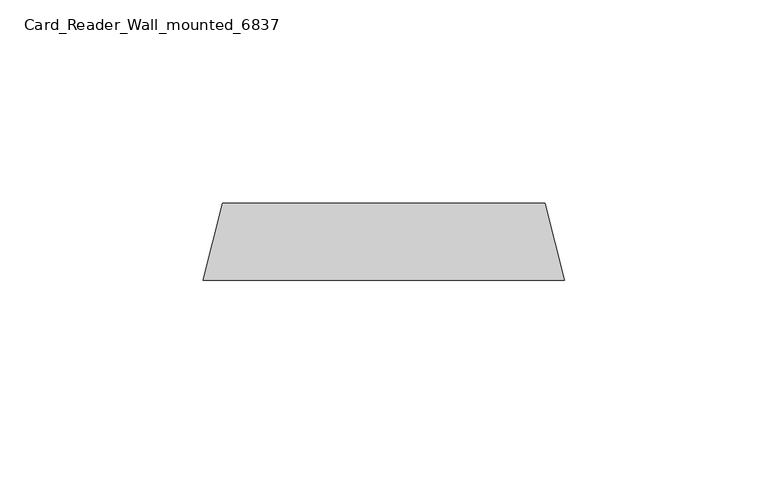
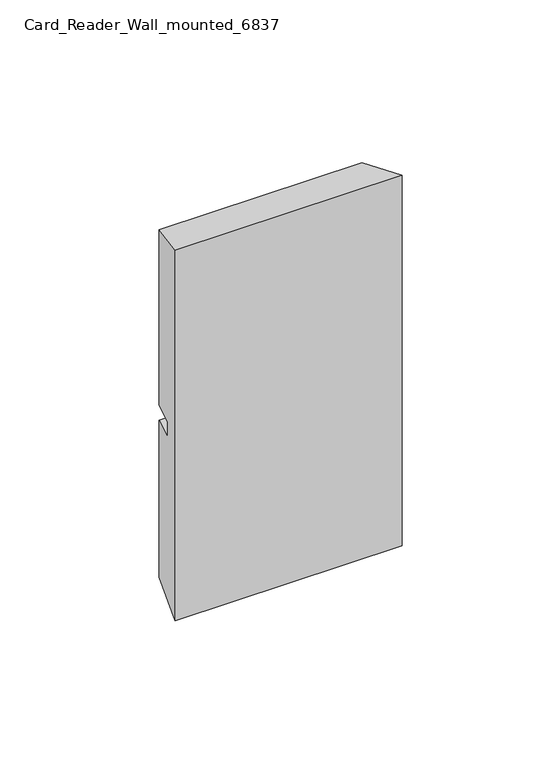
"""IFC4 building model written with IfcOpenShell, lengths in millimetres: proxy geometry, Card_Reader_Wall_mounted_6837 : swipe."""

from ifc_helpers import new_model, si_unit, origin, place, context, project, spatial, faceted_brep, source, transform, mapped, element, save


def card_reader_wall_mounted_6837_593e1b3d(model_context):
    return source(origin(), model_context, "Body", "Brep", [
        faceted_brep([(20.6375, 196.4674974, 1265.2375), (100.0125, 196.4674974, 1265.2375), (100.0125, 196.4674974, 1192.6911313), (20.6375, 196.4674974, 1192.6911313), (100.0125, 196.4674974, 1121.2536313), (20.6375, 196.4674974, 1121.2536313), (20.6375, 196.4674974, 1186.3411313), (100.0125, 196.4674974, 1186.3411313), (15.875, 177.528221, 1270.0), (15.875, 177.528221, 1116.4911313), (104.775, 177.528221, 1116.4911313), (104.775, 177.528221, 1270.0), (102.4977808, 186.5841544, 1186.3411313), (102.4977808, 186.5841544, 1192.6911313), (18.1522192, 186.5841544, 1192.6911313), (18.1522192, 186.5841544, 1186.3411313)], [[[0, 1, 2, 3]], [[4, 5, 6, 7]], [[8, 9, 10, 11]], [[1, 0, 8, 11]], [[11, 10, 4, 7, 12, 13, 2, 1]], [[5, 4, 10, 9]], [[9, 8, 0, 3, 14, 15, 6, 5]], [[14, 13, 12, 15]], [[15, 12, 7, 6]], [[13, 14, 3, 2]]]),
    ])


if __name__ == "__main__":
    model = new_model("IFC4")
    model_context = context("Model", 3, world=origin())
    ifc_project = project(units=[si_unit("LENGTHUNIT", "METRE", prefix="MILLI")], contexts=[model_context])
    site = spatial("IfcSite", under=ifc_project)
    building = spatial("IfcBuilding", under=site)
    placement = place(None, origin())
    card_reader_wall_mounted_6837_shape = card_reader_wall_mounted_6837_593e1b3d(model_context)
    element("IfcBuildingElementProxy", 1, Name="Card_Reader_Wall_mounted_6837 : swipe", ObjectType="Card_Reader_Wall_mounted_6837 : swipe", at=placement, inside=building, context=model_context, shape_type="MappedRepresentation", body=[
        mapped(card_reader_wall_mounted_6837_shape, transform((0.0, 0.0, 0.0), x_axis=(1.0, 0.0, 0.0), y_axis=(0.0, 1.0, 0.0), z_axis=(0.0, 0.0, 1.0))),
    ])
    save(model, "model.ifc")

# Revit data of these elements
# Type "Card_Reader_Wall_mounted_6837 : swipe"
#   COBie.Type.CreatedBy = "design@eagle.com"
#   COBie.Type.CreatedOn = "2016-09-13T05:47:35"
#   COBie.Type.Name = "Security Devices_Card_Reader_Wall_mounted_6837_swipe"
#   COBie.Type.Category = "23-85 30 11 : Access Controls"
#   COBie.Type.Description = ""
#   COBie.Type.Manufacturer = ""
#   COBie.Type.ModelNumber = ""
#   COBie.Type.ReplacementCost = 0
#   Width = 69.85 mm
#   Placement Height = 304.8 mm
#   Height = 114.3 mm
#   COBie.Type = yes
#   Material = Plastic - Black
#   Assembly Code = ""
# Element 1 (IfcBuildingElementProxy, "Card_Reader_Wall_mounted_6837 : swipe")
#   Materials on its faces: "Plastic - Black"
# Materials
#   "Plastic - Black": class "Plastic", colour RGB 0 0 0, transparency 0
